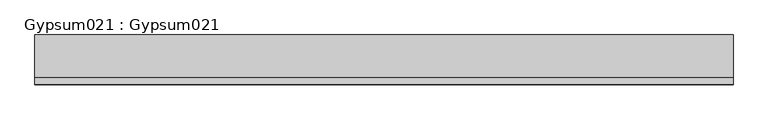
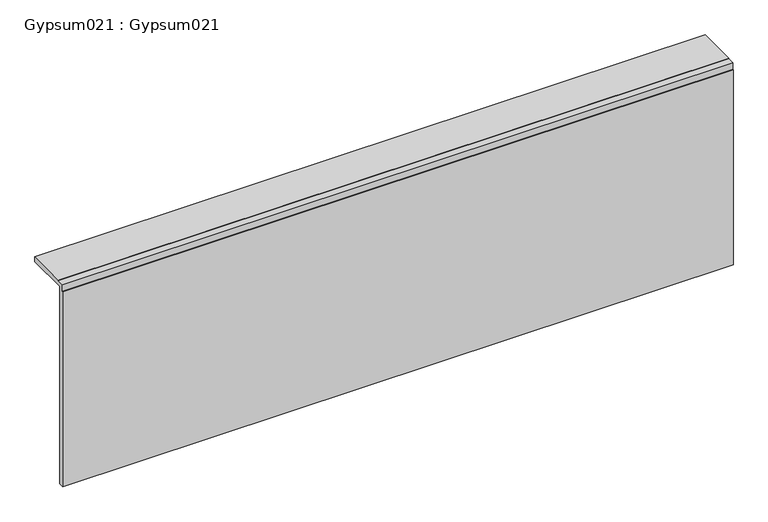
"""IFC4 building model written with IfcOpenShell, lengths in millimetres: proxy geometry, Gypsum021 : Gypsum021."""

from ifc_helpers import new_model, si_unit, frame, origin, place, context, project, spatial, polyline, outline, extrude, source, transform, mapped, element, save


def gypsum021_gypsum021_57715f0e(model_context):
    return source(origin(), model_context, "Body", "SweptSolid", [
        extrude(outline(polyline([(10284.5464235, 40795.72275), (10405.3424948, 40795.72275), (10405.3424948, 40779.84775), (10277.9882396, 40779.84775), (10277.9882396, 40157.1516563), (10262.1132396, 40157.1516563), (10262.1132396, 40773.2895661), (10263.3932396, 40773.2895661), (10263.3932396, 40794.44275), (10284.5464235, 40794.44275), (10284.5464235, 40795.72275)])), frame((3694.2883192, 0.0, 0.0), z_axis=(1.0, 0.0, 0.0), x_axis=(0.0, 1.0, 0.0)), (0.0, 0.0, 1.0), 2000.25),
    ])


if __name__ == "__main__":
    model = new_model("IFC4")
    model_context = context("Model", 3, world=origin())
    ifc_project = project(units=[si_unit("LENGTHUNIT", "METRE", prefix="MILLI")], contexts=[model_context])
    site = spatial("IfcSite", under=ifc_project)
    building = spatial("IfcBuilding", under=site)
    placement = place(None, origin())
    gypsum021_gypsum021_shape = gypsum021_gypsum021_57715f0e(model_context)
    element("IfcBuildingElementProxy", 1, Name="Gypsum021 : Gypsum021", ObjectType="Gypsum021 : Gypsum021", at=placement, inside=building, context=model_context, shape_type="MappedRepresentation", body=[
        mapped(gypsum021_gypsum021_shape, transform((0.0, 0.0, 0.0), x_axis=(1.0, 0.0, 0.0), y_axis=(0.0, 1.0, 0.0), z_axis=(0.0, 0.0, 1.0))),
    ])
    save(model, "model.ifc")

# Revit data of these elements
# Type "Gypsum021 : Gypsum021"
#   NameOverride = "Gypsum021"
# Element 1 (IfcBuildingElementProxy, "Gypsum021 : Gypsum021")
#   Materials on its faces: "5/8\" GYPSUM BOARD"
# Materials
#   "5/8\" GYPSUM BOARD": class "Unassigned", colour RGB 214 214 214, transparency 0, Cost = 0
